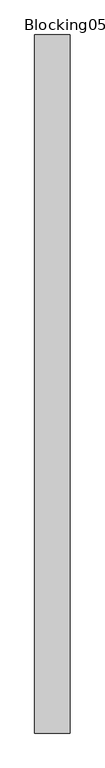
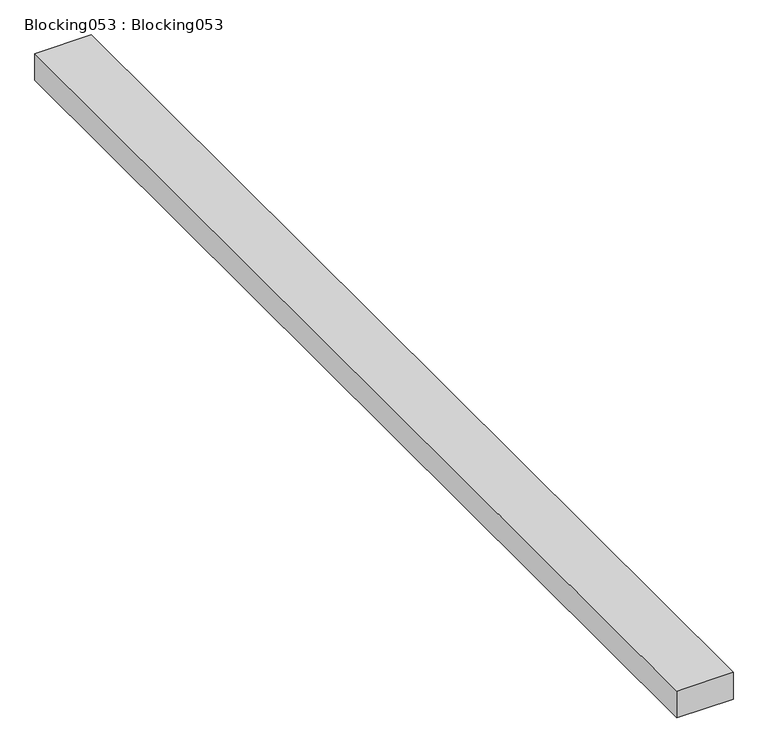
"""IFC4 building model written with IfcOpenShell, lengths in millimetres: proxy geometry, Blocking053 : Blocking053."""

import ifcopenshell
import ifcopenshell.guid

model = None  # the IFC model being written
_history = None  # IfcOwnerHistory: only IFC2X3 demands one
_inside = {}  # id of a spatial element -> (the spatial element, [elements in it])
_under = {}  # id of a project, library or spatial element -> (it, [spatial elements below it])
_declared = {}  # id of a project -> (the project, [libraries it declares])
_typed = {}  # id of a type object -> (the type object, [elements of that type])
_made_of = {}  # id of a material, layer set ... -> (it, [elements and type objects made of it])


def new_model(schema):
    """Start an empty IFC model of exactly this schema.

    Asked for "IFC4X3", IfcOpenShell would pick the latest addendum, in which some entities
    have other attributes; the version numbers below select the first issue.
    IFC2X3 requires an IfcOwnerHistory on every rooted entity: one is made here for all.
    """
    global model, _history
    if schema == "IFC4X3":
        model = ifcopenshell.file(schema_version=(4, 3, 0, 0))
    else:
        model = ifcopenshell.file(schema=schema)
    _inside.clear()
    _under.clear()
    _declared.clear()
    _typed.clear()
    _made_of.clear()
    _history = None
    if model.schema == "IFC2X3":
        org = make("IfcOrganization", Name="unknown")
        user = make(
            "IfcPersonAndOrganization",
            ThePerson=make("IfcPerson", FamilyName="unknown"),
            TheOrganization=org,
        )
        app = make(
            "IfcApplication",
            ApplicationDeveloper=org,
            Version="unknown",
            ApplicationFullName="unknown",
            ApplicationIdentifier="unknown",
        )
        _history = make(
            "IfcOwnerHistory",
            OwningUser=user,
            OwningApplication=app,
            ChangeAction="ADDED",
            CreationDate=0,
        )
    return model


def make(cls, **values):
    """One entity of the class cls with the attributes given. An attribute that is None is left unset."""
    return model.create_entity(
        cls, **{name: value for name, value in values.items() if value is not None}
    )


def rooted(cls, **values):
    """An entity with a GlobalId (a new one), such as an element, a storey or a relation."""
    return make(cls, GlobalId=ifcopenshell.guid.new(), OwnerHistory=_history, **values)


def si_unit(unit_type, name, prefix=None):
    """IfcSIUnit, for example si_unit("LENGTHUNIT", "METRE", prefix="MILLI")."""
    return make("IfcSIUnit", UnitType=unit_type, Prefix=prefix, Name=name)


def assignment(units):
    """IfcUnitAssignment: the units of a project."""
    return None if units is None else make("IfcUnitAssignment", Units=units)


def point(xyz):
    """IfcCartesianPoint."""
    return None if xyz is None else make("IfcCartesianPoint", Coordinates=xyz)


def direction(xyz):
    """IfcDirection."""
    return None if xyz is None else make("IfcDirection", DirectionRatios=xyz)


def frame(location, z_axis=None, x_axis=None):
    """IfcAxis2Placement3D, a coordinate frame: its origin and axes. An axis left out is left unset."""
    return make(
        "IfcAxis2Placement3D",
        Location=point(location),
        Axis=direction(z_axis),
        RefDirection=direction(x_axis),
    )


def origin():
    """The frame at (0, 0, 0) with its axes left unset."""
    return frame((0.0, 0.0, 0.0))


def place(relative_to, where):
    """IfcLocalPlacement: puts the frame where relative to a parent placement (None: the world)."""
    return make(
        "IfcLocalPlacement", PlacementRelTo=relative_to, RelativePlacement=where
    )


def context(
    kind, dimensions, precision=None, world=None, true_north=None, identifier=None
):
    """IfcGeometricRepresentationContext, for example the 3D "Model" context."""
    return make(
        "IfcGeometricRepresentationContext",
        ContextIdentifier=identifier,
        ContextType=kind,
        CoordinateSpaceDimension=dimensions,
        Precision=precision,
        WorldCoordinateSystem=world,
        TrueNorth=true_north,
    )


def project(units=None, contexts=None):
    """IfcProject with its units and contexts."""
    return rooted(
        "IfcProject",
        Name="project",
        RepresentationContexts=contexts,
        UnitsInContext=assignment(units),
    )


def spatial(cls, under=None, at=None, **own):
    """A site, building, storey or space (cls), placed at a placement, below another one or the project."""
    s = rooted(cls, ObjectPlacement=at, **own)
    if under is not None:
        _under.setdefault(under.id(), (under, []))[1].append(s)
    return s


def polyline(points):
    """IfcPolyline through the points."""
    return make("IfcPolyline", Points=[point(p) for p in points])


def outline(outer, holes=None, kind="AREA"):
    """IfcArbitraryClosedProfileDef: a profile drawn as a closed curve; with holes, ...WithVoids."""
    if holes is None:
        return make("IfcArbitraryClosedProfileDef", ProfileType=kind, OuterCurve=outer)
    return make(
        "IfcArbitraryProfileDefWithVoids",
        ProfileType=kind,
        OuterCurve=outer,
        InnerCurves=holes,
    )


def extrude(swept, where, along, depth):
    """IfcExtrudedAreaSolid: the profile swept, set in the frame where, extruded along a direction by depth."""
    return make(
        "IfcExtrudedAreaSolid",
        SweptArea=swept,
        Position=where,
        ExtrudedDirection=direction(along),
        Depth=depth,
    )


def shape(context_of_items, identifier, shape_type, items):
    """IfcShapeRepresentation: the items that make up one representation, for example the "Body"."""
    return make(
        "IfcShapeRepresentation",
        ContextOfItems=context_of_items,
        RepresentationIdentifier=identifier,
        RepresentationType=shape_type,
        Items=items,
    )


def source(mapping_origin, context_of_items, identifier, shape_type, items):
    """IfcRepresentationMap: a shape defined once, which mapped items show again and again."""
    return make(
        "IfcRepresentationMap",
        MappingOrigin=mapping_origin,
        MappedRepresentation=shape(context_of_items, identifier, shape_type, items),
    )


def transform(
    local_origin,
    x_axis=None,
    y_axis=None,
    z_axis=None,
    scale=None,
    scale2=None,
    scale3=None,
    uniform=True,
):
    """IfcCartesianTransformationOperator3D, or its non-uniform kind. x_axis, y_axis, z_axis: its Axis1, 2, 3."""
    if uniform:
        return make(
            "IfcCartesianTransformationOperator3D",
            Axis1=direction(x_axis),
            Axis2=direction(y_axis),
            LocalOrigin=point(local_origin),
            Scale=scale,
            Axis3=direction(z_axis),
        )
    return make(
        "IfcCartesianTransformationOperator3DnonUniform",
        Axis1=direction(x_axis),
        Axis2=direction(y_axis),
        LocalOrigin=point(local_origin),
        Scale=scale,
        Axis3=direction(z_axis),
        Scale2=scale2,
        Scale3=scale3,
    )


def mapped(mapping_source, mapping_target):
    """IfcMappedItem: shows the shape of a source again, moved by a transform."""
    return make(
        "IfcMappedItem", MappingSource=mapping_source, MappingTarget=mapping_target
    )


def made_of(thing, what):
    """Note that an element or type object is made of a material, layer set ...; save() writes the relation."""
    if what is not None:
        _made_of.setdefault(what.id(), (what, []))[1].append(thing)
    return thing


def element(
    cls,
    number,
    at=None,
    inside=None,
    cuts=None,
    type_object=None,
    material=None,
    context=None,
    identifier="Body",
    shape_type=None,
    held_by="IfcProductDefinitionShape",
    body=None,
    shapes=None,
    **own,
):
    """One element of the class cls, such as IfcWall. Its Tag is "e" and its number.

    at: its placement. inside: the storey or other place that contains it. cuts: it is an
    opening in that element (IfcRelVoidsElement). A single representation is given by context,
    identifier, shape_type and body (its items); several are given by shapes. held_by: the class
    of the entity that holds the representations. save() writes the other relations.
    """
    e = rooted(cls, Tag="e%d" % number, ObjectPlacement=at, **own)
    if body is not None:
        shapes = [shape(context, identifier, shape_type, body)]
    if shapes is not None:
        e.Representation = make(held_by, Representations=shapes)
    if inside is not None:
        _inside.setdefault(inside.id(), (inside, []))[1].append(e)
    if cuts is not None:
        rooted(
            "IfcRelVoidsElement", RelatingBuildingElement=cuts, RelatedOpeningElement=e
        )
    if type_object is not None:
        _typed.setdefault(type_object.id(), (type_object, []))[1].append(e)
    return made_of(e, material)


def aggregate(whole, parts):
    """IfcRelAggregates: a whole, such as a stair, and the parts it consists of."""
    return rooted("IfcRelAggregates", RelatingObject=whole, RelatedObjects=parts)


def save(model, path):
    """Write the relations noted so far, then the file.

    IfcRelAggregates (storeys below a building ...), IfcRelContainedInSpatialStructure (elements
    in a storey), IfcRelDefinesByType, IfcRelAssociatesMaterial and IfcRelDeclares: one each for
    every whole, place, type object, material and project.
    """
    for whole, parts in _under.values():
        aggregate(whole, parts)
    for where, things in _inside.values():
        rooted(
            "IfcRelContainedInSpatialStructure",
            RelatedElements=things,
            RelatingStructure=where,
        )
    for kind, things in _typed.values():
        rooted("IfcRelDefinesByType", RelatedObjects=things, RelatingType=kind)
    for what, things in _made_of.values():
        rooted("IfcRelAssociatesMaterial", RelatedObjects=things, RelatingMaterial=what)
    for by, libraries in _declared.values():
        rooted("IfcRelDeclares", RelatingContext=by, RelatedDefinitions=libraries)
    model.write(path)


def blocking053_blocking053_edcbc8be(model_context):
    return source(origin(), model_context, "Body", "SweptSolid", [
        extrude(outline(polyline([(-9787.3237014, 7982.1531721), (-9888.9237014, 7982.1531721), (-9888.9237014, 9982.1531721), (-9787.3237014, 9982.1531721), (-9787.3237014, 7982.1531721)])), frame((0.0, 0.0, 40055.5460083), z_axis=(0.0, 0.0, 1.0), x_axis=(1.0, 0.0, 0.0)), (0.0, 0.0, 1.0), 50.8),
    ])


if __name__ == "__main__":
    model = new_model("IFC4")
    model_context = context("Model", 3, world=origin())
    ifc_project = project(units=[si_unit("LENGTHUNIT", "METRE", prefix="MILLI")], contexts=[model_context])
    site = spatial("IfcSite", under=ifc_project)
    building = spatial("IfcBuilding", under=site)
    placement = place(None, origin())
    blocking053_blocking053_shape = blocking053_blocking053_edcbc8be(model_context)
    element("IfcBuildingElementProxy", 1, Name="Blocking053 : Blocking053", ObjectType="Blocking053 : Blocking053", at=placement, inside=building, context=model_context, shape_type="MappedRepresentation", body=[
        mapped(blocking053_blocking053_shape, transform((0.0, 0.0, 0.0), x_axis=(1.0, 0.0, 0.0), y_axis=(0.0, 1.0, 0.0), z_axis=(0.0, 0.0, 1.0))),
    ])
    save(model, "model.ifc")

# Revit data of these elements
# Type "Blocking053 : Blocking053"
#   NameOverride = "Blocking053"
# Element 1 (IfcBuildingElementProxy, "Blocking053 : Blocking053")
#   Materials on its faces: "WOOD BLOCKING AS REQUIRED"
# Materials
#   "WOOD BLOCKING AS REQUIRED": class "Unassigned", colour RGB 166 124 85, transparency 0, Cost = 0
